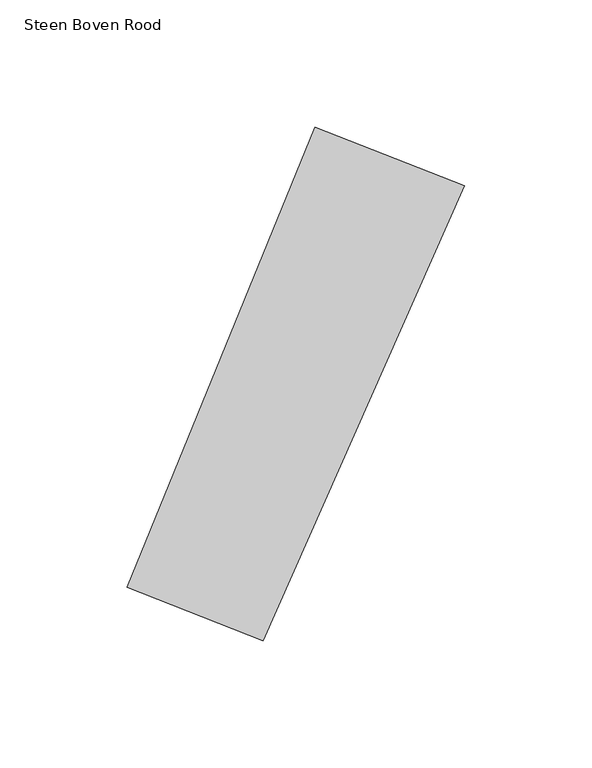
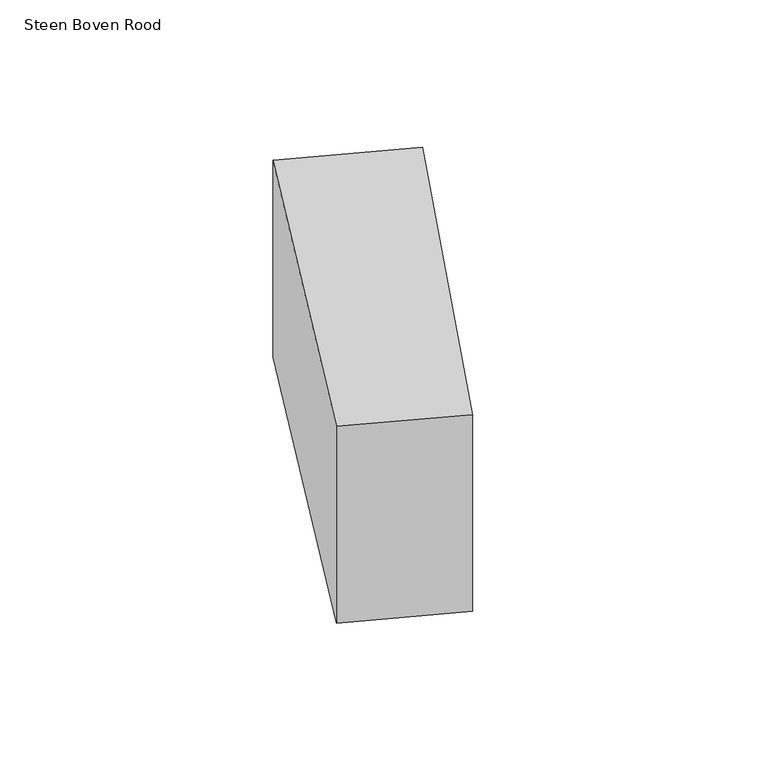
"""IFC4 building model written with IfcOpenShell, lengths in millimetres: proxy geometry, 00_GMA_steen_versie_4 : Steen Boven Rood."""

import ifcopenshell
import ifcopenshell.guid

model = None  # the IFC model being written
_history = None  # IfcOwnerHistory: only IFC2X3 demands one
_inside = {}  # id of a spatial element -> (the spatial element, [elements in it])
_under = {}  # id of a project, library or spatial element -> (it, [spatial elements below it])
_declared = {}  # id of a project -> (the project, [libraries it declares])
_typed = {}  # id of a type object -> (the type object, [elements of that type])
_made_of = {}  # id of a material, layer set ... -> (it, [elements and type objects made of it])


def new_model(schema):
    """Start an empty IFC model of exactly this schema.

    Asked for "IFC4X3", IfcOpenShell would pick the latest addendum, in which some entities
    have other attributes; the version numbers below select the first issue.
    IFC2X3 requires an IfcOwnerHistory on every rooted entity: one is made here for all.
    """
    global model, _history
    if schema == "IFC4X3":
        model = ifcopenshell.file(schema_version=(4, 3, 0, 0))
    else:
        model = ifcopenshell.file(schema=schema)
    _inside.clear()
    _under.clear()
    _declared.clear()
    _typed.clear()
    _made_of.clear()
    _history = None
    if model.schema == "IFC2X3":
        org = make("IfcOrganization", Name="unknown")
        user = make(
            "IfcPersonAndOrganization",
            ThePerson=make("IfcPerson", FamilyName="unknown"),
            TheOrganization=org,
        )
        app = make(
            "IfcApplication",
            ApplicationDeveloper=org,
            Version="unknown",
            ApplicationFullName="unknown",
            ApplicationIdentifier="unknown",
        )
        _history = make(
            "IfcOwnerHistory",
            OwningUser=user,
            OwningApplication=app,
            ChangeAction="ADDED",
            CreationDate=0,
        )
    return model


def make(cls, **values):
    """One entity of the class cls with the attributes given. An attribute that is None is left unset."""
    return model.create_entity(
        cls, **{name: value for name, value in values.items() if value is not None}
    )


def rooted(cls, **values):
    """An entity with a GlobalId (a new one), such as an element, a storey or a relation."""
    return make(cls, GlobalId=ifcopenshell.guid.new(), OwnerHistory=_history, **values)


def si_unit(unit_type, name, prefix=None):
    """IfcSIUnit, for example si_unit("LENGTHUNIT", "METRE", prefix="MILLI")."""
    return make("IfcSIUnit", UnitType=unit_type, Prefix=prefix, Name=name)


def assignment(units):
    """IfcUnitAssignment: the units of a project."""
    return None if units is None else make("IfcUnitAssignment", Units=units)


def point(xyz):
    """IfcCartesianPoint."""
    return None if xyz is None else make("IfcCartesianPoint", Coordinates=xyz)


def direction(xyz):
    """IfcDirection."""
    return None if xyz is None else make("IfcDirection", DirectionRatios=xyz)


def frame(location, z_axis=None, x_axis=None):
    """IfcAxis2Placement3D, a coordinate frame: its origin and axes. An axis left out is left unset."""
    return make(
        "IfcAxis2Placement3D",
        Location=point(location),
        Axis=direction(z_axis),
        RefDirection=direction(x_axis),
    )


def origin():
    """The frame at (0, 0, 0) with its axes left unset."""
    return frame((0.0, 0.0, 0.0))


def origin_with_axes():
    """The frame at (0, 0, 0) with the z axis (0, 0, 1) and the x axis (1, 0, 0) written out."""
    return frame((0.0, 0.0, 0.0), z_axis=(0.0, 0.0, 1.0), x_axis=(1.0, 0.0, 0.0))


def place(relative_to, where):
    """IfcLocalPlacement: puts the frame where relative to a parent placement (None: the world)."""
    return make(
        "IfcLocalPlacement", PlacementRelTo=relative_to, RelativePlacement=where
    )


def context(
    kind, dimensions, precision=None, world=None, true_north=None, identifier=None
):
    """IfcGeometricRepresentationContext, for example the 3D "Model" context."""
    return make(
        "IfcGeometricRepresentationContext",
        ContextIdentifier=identifier,
        ContextType=kind,
        CoordinateSpaceDimension=dimensions,
        Precision=precision,
        WorldCoordinateSystem=world,
        TrueNorth=true_north,
    )


def project(units=None, contexts=None):
    """IfcProject with its units and contexts."""
    return rooted(
        "IfcProject",
        Name="project",
        RepresentationContexts=contexts,
        UnitsInContext=assignment(units),
    )


def spatial(cls, under=None, at=None, **own):
    """A site, building, storey or space (cls), placed at a placement, below another one or the project."""
    s = rooted(cls, ObjectPlacement=at, **own)
    if under is not None:
        _under.setdefault(under.id(), (under, []))[1].append(s)
    return s


def polyline(points):
    """IfcPolyline through the points."""
    return make("IfcPolyline", Points=[point(p) for p in points])


def outline(outer, holes=None, kind="AREA"):
    """IfcArbitraryClosedProfileDef: a profile drawn as a closed curve; with holes, ...WithVoids."""
    if holes is None:
        return make("IfcArbitraryClosedProfileDef", ProfileType=kind, OuterCurve=outer)
    return make(
        "IfcArbitraryProfileDefWithVoids",
        ProfileType=kind,
        OuterCurve=outer,
        InnerCurves=holes,
    )


def extrude(swept, where, along, depth):
    """IfcExtrudedAreaSolid: the profile swept, set in the frame where, extruded along a direction by depth."""
    return make(
        "IfcExtrudedAreaSolid",
        SweptArea=swept,
        Position=where,
        ExtrudedDirection=direction(along),
        Depth=depth,
    )


def shape(context_of_items, identifier, shape_type, items):
    """IfcShapeRepresentation: the items that make up one representation, for example the "Body"."""
    return make(
        "IfcShapeRepresentation",
        ContextOfItems=context_of_items,
        RepresentationIdentifier=identifier,
        RepresentationType=shape_type,
        Items=items,
    )


def source(mapping_origin, context_of_items, identifier, shape_type, items):
    """IfcRepresentationMap: a shape defined once, which mapped items show again and again."""
    return make(
        "IfcRepresentationMap",
        MappingOrigin=mapping_origin,
        MappedRepresentation=shape(context_of_items, identifier, shape_type, items),
    )


def transform(
    local_origin,
    x_axis=None,
    y_axis=None,
    z_axis=None,
    scale=None,
    scale2=None,
    scale3=None,
    uniform=True,
):
    """IfcCartesianTransformationOperator3D, or its non-uniform kind. x_axis, y_axis, z_axis: its Axis1, 2, 3."""
    if uniform:
        return make(
            "IfcCartesianTransformationOperator3D",
            Axis1=direction(x_axis),
            Axis2=direction(y_axis),
            LocalOrigin=point(local_origin),
            Scale=scale,
            Axis3=direction(z_axis),
        )
    return make(
        "IfcCartesianTransformationOperator3DnonUniform",
        Axis1=direction(x_axis),
        Axis2=direction(y_axis),
        LocalOrigin=point(local_origin),
        Scale=scale,
        Axis3=direction(z_axis),
        Scale2=scale2,
        Scale3=scale3,
    )


def mapped(mapping_source, mapping_target):
    """IfcMappedItem: shows the shape of a source again, moved by a transform."""
    return make(
        "IfcMappedItem", MappingSource=mapping_source, MappingTarget=mapping_target
    )


def made_of(thing, what):
    """Note that an element or type object is made of a material, layer set ...; save() writes the relation."""
    if what is not None:
        _made_of.setdefault(what.id(), (what, []))[1].append(thing)
    return thing


def element(
    cls,
    number,
    at=None,
    inside=None,
    cuts=None,
    type_object=None,
    material=None,
    context=None,
    identifier="Body",
    shape_type=None,
    held_by="IfcProductDefinitionShape",
    body=None,
    shapes=None,
    **own,
):
    """One element of the class cls, such as IfcWall. Its Tag is "e" and its number.

    at: its placement. inside: the storey or other place that contains it. cuts: it is an
    opening in that element (IfcRelVoidsElement). A single representation is given by context,
    identifier, shape_type and body (its items); several are given by shapes. held_by: the class
    of the entity that holds the representations. save() writes the other relations.
    """
    e = rooted(cls, Tag="e%d" % number, ObjectPlacement=at, **own)
    if body is not None:
        shapes = [shape(context, identifier, shape_type, body)]
    if shapes is not None:
        e.Representation = make(held_by, Representations=shapes)
    if inside is not None:
        _inside.setdefault(inside.id(), (inside, []))[1].append(e)
    if cuts is not None:
        rooted(
            "IfcRelVoidsElement", RelatingBuildingElement=cuts, RelatedOpeningElement=e
        )
    if type_object is not None:
        _typed.setdefault(type_object.id(), (type_object, []))[1].append(e)
    return made_of(e, material)


def aggregate(whole, parts):
    """IfcRelAggregates: a whole, such as a stair, and the parts it consists of."""
    return rooted("IfcRelAggregates", RelatingObject=whole, RelatedObjects=parts)


def save(model, path):
    """Write the relations noted so far, then the file.

    IfcRelAggregates (storeys below a building ...), IfcRelContainedInSpatialStructure (elements
    in a storey), IfcRelDefinesByType, IfcRelAssociatesMaterial and IfcRelDeclares: one each for
    every whole, place, type object, material and project.
    """
    for whole, parts in _under.values():
        aggregate(whole, parts)
    for where, things in _inside.values():
        rooted(
            "IfcRelContainedInSpatialStructure",
            RelatedElements=things,
            RelatingStructure=where,
        )
    for kind, things in _typed.values():
        rooted("IfcRelDefinesByType", RelatedObjects=things, RelatingType=kind)
    for what, things in _made_of.values():
        rooted("IfcRelAssociatesMaterial", RelatedObjects=things, RelatingMaterial=what)
    for by, libraries in _declared.values():
        rooted("IfcRelDeclares", RelatingContext=by, RelatedDefinitions=libraries)
    model.write(path)


def steen_boven_rood_b1bde73d(model_context):
    return source(origin(), model_context, "Body", "SweptSolid", [
        extrude(outline(polyline([(141.4233667, 161.9435257), (62.3950875, -16.5344435), (8.9655103, 4.3789098), (82.6842684, 184.9308384), (141.4233667, 161.9435257)])), origin_with_axes(), (0.0, 0.0, 1.0), 100.0),
    ])


if __name__ == "__main__":
    model = new_model("IFC4")
    model_context = context("Model", 3, world=origin())
    ifc_project = project(units=[si_unit("LENGTHUNIT", "METRE", prefix="MILLI")], contexts=[model_context])
    site = spatial("IfcSite", under=ifc_project)
    building = spatial("IfcBuilding", under=site)
    placement = place(None, origin())
    steen_boven_rood_shape = steen_boven_rood_b1bde73d(model_context)
    element("IfcBuildingElementProxy", 1, Name="00_GMA_steen_versie_4 : Steen Boven Rood", ObjectType="00_GMA_steen_versie_4 : Steen Boven Rood", at=placement, inside=building, context=model_context, shape_type="MappedRepresentation", body=[
        mapped(steen_boven_rood_shape, transform((0.0, 0.0, 0.0), x_axis=(1.0, 0.0, 0.0), y_axis=(0.0, 1.0, 0.0), z_axis=(0.0, 0.0, 1.0))),
    ])
    save(model, "model.ifc")

# Revit data of these elements
# Type "00_GMA_steen_versie_4 : Steen Boven Rood"
#   StootVoegHalfBoven [instance default] = 5 mm
#   StootVoegHalf [instance default] = 5 mm
#   StootVoegBreedteOnder = 10 mm
#   StootVoegBreedteBoven = 10 mm
#   Steendikte = 100 mm
#   LintVoegOnderHalf = 5 mm
#   LintVoegOnder = 10 mm
#   LintVoegBovenHalf = 0 mm
#   LintVoegBoven = 0 mm
#   materiaal = 21_steen_rood
#   MateriaalVoeg = none
#   Default Elevation = 0
# Element 1 (IfcBuildingElementProxy, "00_GMA_steen_versie_4 : Steen Boven Rood")
#   Materials on its faces: "21_steen_rood"
# Materials
#   "21_steen_rood": class "Unassigned", colour RGB 213 111 43, transparency 0, Cost = 0
